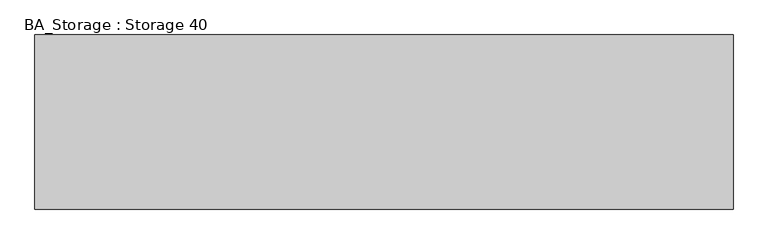
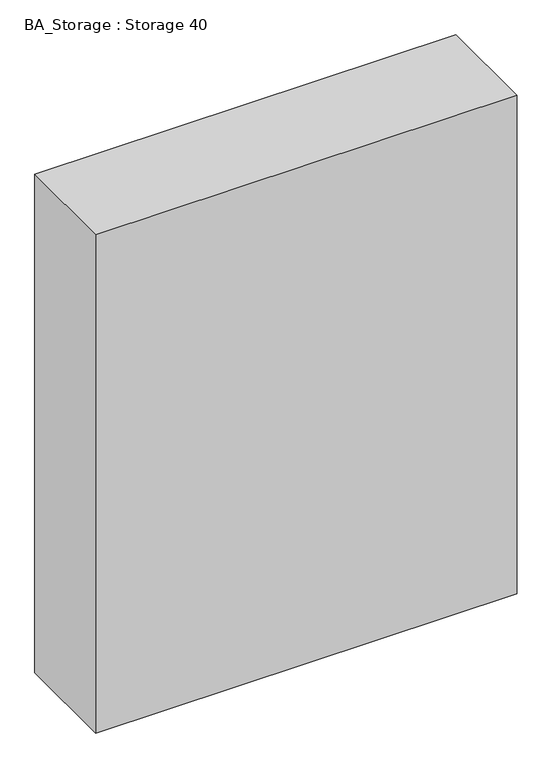
"""IFC4 building model written with IfcOpenShell, lengths in millimetres: furniture geometry, BA_Storage : Storage 40."""

from ifc_helpers import new_model, si_unit, origin, origin_with_axes, place, context, project, spatial, polyline, outline, extrude, source, transform, mapped, element, save


def ba_storage_storage_40_0585c1d1(model_context):
    return source(origin(), model_context, "Body", "SweptSolid", [
        extrude(outline(polyline([(1600.0, 0.0), (1600.0, -400.0), (0.0, -400.0), (0.0, 0.0), (1600.0, 0.0)])), origin_with_axes(), (0.0, 0.0, 1.0), 2000.0),
    ])


if __name__ == "__main__":
    model = new_model("IFC4")
    model_context = context("Model", 3, world=origin())
    ifc_project = project(units=[si_unit("LENGTHUNIT", "METRE", prefix="MILLI")], contexts=[model_context])
    site = spatial("IfcSite", under=ifc_project)
    building = spatial("IfcBuilding", under=site)
    placement = place(None, origin())
    ba_storage_storage_40_shape = ba_storage_storage_40_0585c1d1(model_context)
    element("IfcFurniture", 1, ObjectType="BA_Storage : Storage 40", at=placement, inside=building, context=model_context, shape_type="MappedRepresentation", body=[
        mapped(ba_storage_storage_40_shape, transform((0.0, 0.0, 0.0), x_axis=(1.0, 0.0, 0.0), y_axis=(0.0, 1.0, 0.0), z_axis=(0.0, 0.0, 1.0))),
    ])
    save(model, "model.ifc")

# Revit data of these elements
# Type "BA_Storage : Storage 40"
#   built-in parameter 1001306 [instance default] = 4.85564 (stored number, unit not read)
#   Height [instance default] = 2000 mm
#   depth = 400 mm
#   Default Elevation = 0
# Element 1 (IfcFurniture, "BA_Storage : Storage 40")
#   built-in parameter 1001306 = 5.24934 (stored number, unit not read)
#   Materials on its faces: "Default"
# Materials
#   "Default": class "Generic", colour RGB 255 255 255, transparency 0, Cost = 0
